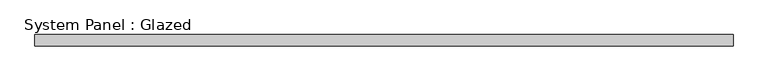
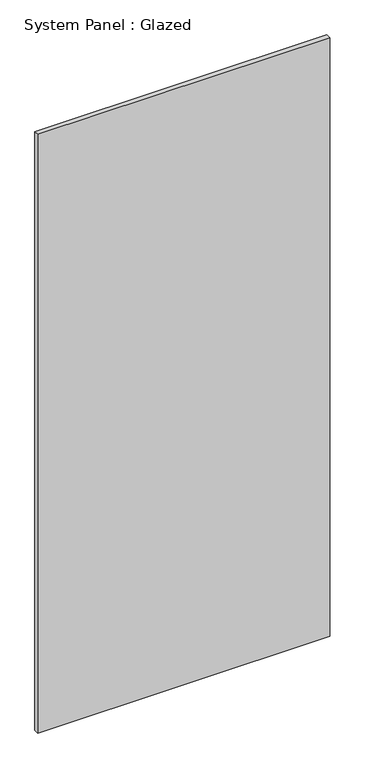
"""IFC4 building model written with IfcOpenShell, lengths in millimetres: plate geometry, System Panel : Glazed."""

from ifc_helpers import new_model, si_unit, origin, origin_with_axes, place, context, project, spatial, polyline, outline, extrude, source, transform, mapped, element, save


def system_panel_glazed_ff630af2(model_context):
    return source(origin(), model_context, "Body", "SweptSolid", [
        extrude(outline(polyline([(796.9250048, 19.05), (-796.9250048, 19.05), (-796.9250048, 44.45), (796.9250048, 44.45), (796.9250048, 19.05)])), origin_with_axes(), (0.0, 0.0, 1.0), 3454.4),
    ])


if __name__ == "__main__":
    model = new_model("IFC4")
    model_context = context("Model", 3, world=origin())
    ifc_project = project(units=[si_unit("LENGTHUNIT", "METRE", prefix="MILLI")], contexts=[model_context])
    site = spatial("IfcSite", under=ifc_project)
    building = spatial("IfcBuilding", under=site)
    placement = place(None, origin())
    system_panel_glazed_shape = system_panel_glazed_ff630af2(model_context)
    element("IfcPlate", 1, ObjectType="System Panel : Glazed", at=placement, inside=building, context=model_context, shape_type="MappedRepresentation", body=[
        mapped(system_panel_glazed_shape, transform((0.0, 0.0, 0.0), x_axis=(1.0, 0.0, 0.0), y_axis=(0.0, 1.0, 0.0), z_axis=(0.0, 0.0, 1.0))),
    ])
    save(model, "model.ifc")

# Revit data of these elements
# Type "System Panel : Glazed"
#   Construction Type Id = "GSP4R"
#   Analytic Construction = "1/8 in Pilkington single glazing"
#   Visual Light Transmittance = 0.9
#   Solar Heat Gain Coefficient = 0.86
#   Heat Transfer Coefficient (U) = 1.18115 BTU/(h·ft²·°F)
#   Define Thermal Properties by = 1
# Element 1 (IfcPlate, "System Panel : Glazed")
#   Materials on its faces: "Glass"
# Materials
#   "Glass": class "Glass", colour RGB 0 128 192, transparency 0.75, Description = "Soda Lime Glass", Cost = 0
